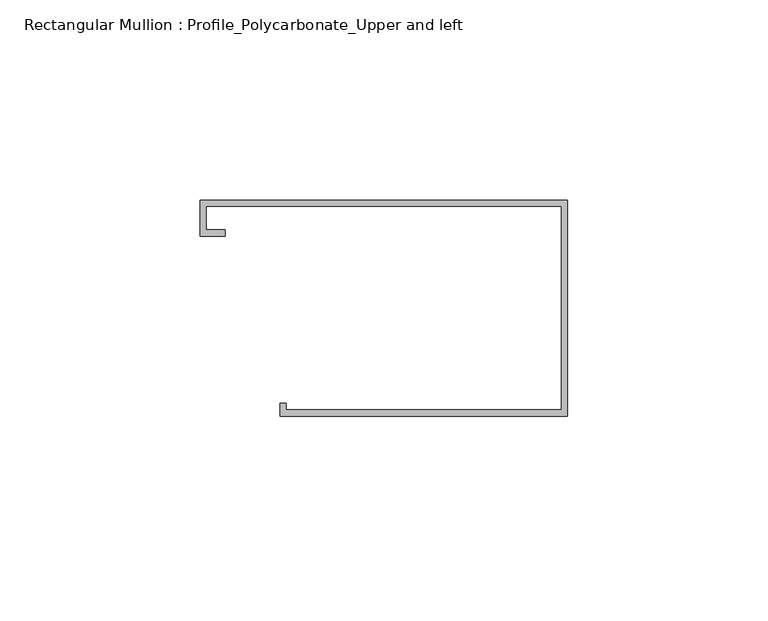
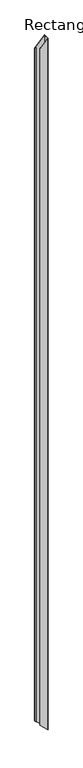
"""IFC4 building model written with IfcOpenShell, lengths in millimetres: member geometry, Rectangular Mullion : Profile_Polycarbonate_Upper and left."""

from ifc_helpers import new_model, si_unit, origin, place, context, project, spatial, faceted_brep, source, transform, mapped, element, save


def rectangular_mullion_profile_polycarbonate_upper_and_left_103d42f7(model_context):
    return source(origin(), model_context, "Body", "Brep", [
        faceted_brep([(-91.9988, 28.984575, -95.9119088), (0.0, 28.984575, 0.0), (0.0, 28.984575, -6723.0017223), (-91.9988, 28.984575, -6634.7563802), (-91.9988, 19.992975, -95.9119088), (-91.9988, 19.992975, -6634.7563802), (-85.6488, 19.992975, -89.2918157), (-85.6488, 19.992975, -6640.8473066), (-85.6488, 21.580475, -89.2918157), (-85.6488, 21.580475, -6640.8473066), (-90.4113, 21.580475, -94.2568855), (-90.4113, 21.580475, -6636.2791118), (-90.4113, 27.397075, -94.2568855), (-90.4113, 27.397075, -6636.2791118), (-1.5875, 27.397075, -1.6550233), (-1.5875, 27.397075, -6721.4789907), (-1.5875, -23.428325, -1.6550233), (-1.5875, -23.428325, -6721.4789907), (-70.3961, -23.428325, -73.3903521), (-70.3961, -23.428325, -6655.4777119), (-70.3961, -21.840825, -73.3903521), (-70.3961, -21.840825, -6655.4777119), (-71.9836, -21.840825, -75.0453753), (-71.9836, -21.840825, -6653.9549803), (-71.9836, -25.015825, -75.0453753), (-71.9836, -25.015825, -6653.9549803), (0.0, -25.015825, 0.0), (0.0, -25.015825, -6723.0017223)], [[[0, 1, 2, 3]], [[4, 0, 3, 5]], [[6, 4, 5, 7]], [[8, 6, 7, 9]], [[10, 8, 9, 11]], [[12, 10, 11, 13]], [[14, 12, 13, 15]], [[16, 14, 15, 17]], [[18, 16, 17, 19]], [[20, 18, 19, 21]], [[22, 20, 21, 23]], [[24, 22, 23, 25]], [[26, 24, 25, 27]], [[1, 26, 27, 2]], [[1, 0, 4, 6, 8, 10, 12, 14, 16, 18, 20, 22, 24, 26]], [[2, 27, 25, 23, 21, 19, 17, 15, 13, 11, 9, 7, 5, 3]]]),
    ])


if __name__ == "__main__":
    model = new_model("IFC4")
    model_context = context("Model", 3, world=origin())
    ifc_project = project(units=[si_unit("LENGTHUNIT", "METRE", prefix="MILLI")], contexts=[model_context])
    site = spatial("IfcSite", under=ifc_project)
    building = spatial("IfcBuilding", under=site)
    placement = place(None, origin())
    rectangular_mullion_profile_polycarbonate_upper_and_left_shape = rectangular_mullion_profile_polycarbonate_upper_and_left_103d42f7(model_context)
    element("IfcMember", 1, ObjectType="Rectangular Mullion : Profile_Polycarbonate_Upper and left", at=placement, inside=building, context=model_context, shape_type="MappedRepresentation", body=[
        mapped(rectangular_mullion_profile_polycarbonate_upper_and_left_shape, transform((0.0, 0.0, 0.0), x_axis=(1.0, 0.0, 0.0), y_axis=(0.0, 1.0, 0.0), z_axis=(0.0, 0.0, 1.0))),
    ])
    save(model, "model.ifc")

# Revit data of these elements
# Type "Rectangular Mullion : Profile_Polycarbonate_Upper and left"
#   built-in parameter 1007322 = 0.177167 (stored number, unit not read)
#   built-in parameter 1007321 = 0.00520833 (stored number, unit not read)
#   built-in parameter 1007320 = 0 (stored number, unit not read)
